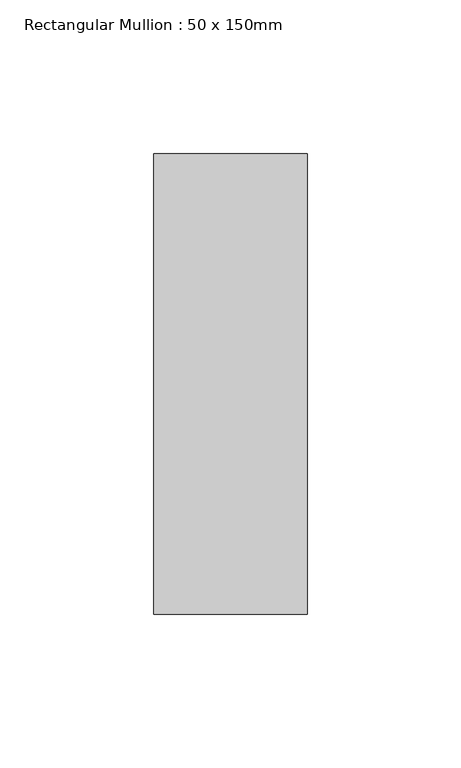
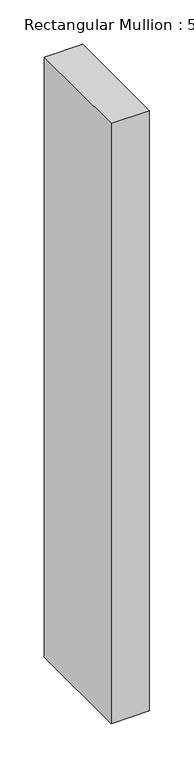
"""IFC4 building model written with IfcOpenShell, lengths in millimetres: member geometry, Rectangular Mullion : 50 x 150mm."""

import ifcopenshell
import ifcopenshell.guid

model = None  # the IFC model being written
_history = None  # IfcOwnerHistory: only IFC2X3 demands one
_inside = {}  # id of a spatial element -> (the spatial element, [elements in it])
_under = {}  # id of a project, library or spatial element -> (it, [spatial elements below it])
_declared = {}  # id of a project -> (the project, [libraries it declares])
_typed = {}  # id of a type object -> (the type object, [elements of that type])
_made_of = {}  # id of a material, layer set ... -> (it, [elements and type objects made of it])


def new_model(schema):
    """Start an empty IFC model of exactly this schema.

    Asked for "IFC4X3", IfcOpenShell would pick the latest addendum, in which some entities
    have other attributes; the version numbers below select the first issue.
    IFC2X3 requires an IfcOwnerHistory on every rooted entity: one is made here for all.
    """
    global model, _history
    if schema == "IFC4X3":
        model = ifcopenshell.file(schema_version=(4, 3, 0, 0))
    else:
        model = ifcopenshell.file(schema=schema)
    _inside.clear()
    _under.clear()
    _declared.clear()
    _typed.clear()
    _made_of.clear()
    _history = None
    if model.schema == "IFC2X3":
        org = make("IfcOrganization", Name="unknown")
        user = make(
            "IfcPersonAndOrganization",
            ThePerson=make("IfcPerson", FamilyName="unknown"),
            TheOrganization=org,
        )
        app = make(
            "IfcApplication",
            ApplicationDeveloper=org,
            Version="unknown",
            ApplicationFullName="unknown",
            ApplicationIdentifier="unknown",
        )
        _history = make(
            "IfcOwnerHistory",
            OwningUser=user,
            OwningApplication=app,
            ChangeAction="ADDED",
            CreationDate=0,
        )
    return model


def make(cls, **values):
    """One entity of the class cls with the attributes given. An attribute that is None is left unset."""
    return model.create_entity(
        cls, **{name: value for name, value in values.items() if value is not None}
    )


def rooted(cls, **values):
    """An entity with a GlobalId (a new one), such as an element, a storey or a relation."""
    return make(cls, GlobalId=ifcopenshell.guid.new(), OwnerHistory=_history, **values)


def si_unit(unit_type, name, prefix=None):
    """IfcSIUnit, for example si_unit("LENGTHUNIT", "METRE", prefix="MILLI")."""
    return make("IfcSIUnit", UnitType=unit_type, Prefix=prefix, Name=name)


def assignment(units):
    """IfcUnitAssignment: the units of a project."""
    return None if units is None else make("IfcUnitAssignment", Units=units)


def point(xyz):
    """IfcCartesianPoint."""
    return None if xyz is None else make("IfcCartesianPoint", Coordinates=xyz)


def direction(xyz):
    """IfcDirection."""
    return None if xyz is None else make("IfcDirection", DirectionRatios=xyz)


def frame(location, z_axis=None, x_axis=None):
    """IfcAxis2Placement3D, a coordinate frame: its origin and axes. An axis left out is left unset."""
    return make(
        "IfcAxis2Placement3D",
        Location=point(location),
        Axis=direction(z_axis),
        RefDirection=direction(x_axis),
    )


def origin():
    """The frame at (0, 0, 0) with its axes left unset."""
    return frame((0.0, 0.0, 0.0))


def place(relative_to, where):
    """IfcLocalPlacement: puts the frame where relative to a parent placement (None: the world)."""
    return make(
        "IfcLocalPlacement", PlacementRelTo=relative_to, RelativePlacement=where
    )


def context(
    kind, dimensions, precision=None, world=None, true_north=None, identifier=None
):
    """IfcGeometricRepresentationContext, for example the 3D "Model" context."""
    return make(
        "IfcGeometricRepresentationContext",
        ContextIdentifier=identifier,
        ContextType=kind,
        CoordinateSpaceDimension=dimensions,
        Precision=precision,
        WorldCoordinateSystem=world,
        TrueNorth=true_north,
    )


def project(units=None, contexts=None):
    """IfcProject with its units and contexts."""
    return rooted(
        "IfcProject",
        Name="project",
        RepresentationContexts=contexts,
        UnitsInContext=assignment(units),
    )


def spatial(cls, under=None, at=None, **own):
    """A site, building, storey or space (cls), placed at a placement, below another one or the project."""
    s = rooted(cls, ObjectPlacement=at, **own)
    if under is not None:
        _under.setdefault(under.id(), (under, []))[1].append(s)
    return s


def polyline(points):
    """IfcPolyline through the points."""
    return make("IfcPolyline", Points=[point(p) for p in points])


def outline(outer, holes=None, kind="AREA"):
    """IfcArbitraryClosedProfileDef: a profile drawn as a closed curve; with holes, ...WithVoids."""
    if holes is None:
        return make("IfcArbitraryClosedProfileDef", ProfileType=kind, OuterCurve=outer)
    return make(
        "IfcArbitraryProfileDefWithVoids",
        ProfileType=kind,
        OuterCurve=outer,
        InnerCurves=holes,
    )


def extrude(swept, where, along, depth):
    """IfcExtrudedAreaSolid: the profile swept, set in the frame where, extruded along a direction by depth."""
    return make(
        "IfcExtrudedAreaSolid",
        SweptArea=swept,
        Position=where,
        ExtrudedDirection=direction(along),
        Depth=depth,
    )


def shape(context_of_items, identifier, shape_type, items):
    """IfcShapeRepresentation: the items that make up one representation, for example the "Body"."""
    return make(
        "IfcShapeRepresentation",
        ContextOfItems=context_of_items,
        RepresentationIdentifier=identifier,
        RepresentationType=shape_type,
        Items=items,
    )


def source(mapping_origin, context_of_items, identifier, shape_type, items):
    """IfcRepresentationMap: a shape defined once, which mapped items show again and again."""
    return make(
        "IfcRepresentationMap",
        MappingOrigin=mapping_origin,
        MappedRepresentation=shape(context_of_items, identifier, shape_type, items),
    )


def transform(
    local_origin,
    x_axis=None,
    y_axis=None,
    z_axis=None,
    scale=None,
    scale2=None,
    scale3=None,
    uniform=True,
):
    """IfcCartesianTransformationOperator3D, or its non-uniform kind. x_axis, y_axis, z_axis: its Axis1, 2, 3."""
    if uniform:
        return make(
            "IfcCartesianTransformationOperator3D",
            Axis1=direction(x_axis),
            Axis2=direction(y_axis),
            LocalOrigin=point(local_origin),
            Scale=scale,
            Axis3=direction(z_axis),
        )
    return make(
        "IfcCartesianTransformationOperator3DnonUniform",
        Axis1=direction(x_axis),
        Axis2=direction(y_axis),
        LocalOrigin=point(local_origin),
        Scale=scale,
        Axis3=direction(z_axis),
        Scale2=scale2,
        Scale3=scale3,
    )


def mapped(mapping_source, mapping_target):
    """IfcMappedItem: shows the shape of a source again, moved by a transform."""
    return make(
        "IfcMappedItem", MappingSource=mapping_source, MappingTarget=mapping_target
    )


def made_of(thing, what):
    """Note that an element or type object is made of a material, layer set ...; save() writes the relation."""
    if what is not None:
        _made_of.setdefault(what.id(), (what, []))[1].append(thing)
    return thing


def element(
    cls,
    number,
    at=None,
    inside=None,
    cuts=None,
    type_object=None,
    material=None,
    context=None,
    identifier="Body",
    shape_type=None,
    held_by="IfcProductDefinitionShape",
    body=None,
    shapes=None,
    **own,
):
    """One element of the class cls, such as IfcWall. Its Tag is "e" and its number.

    at: its placement. inside: the storey or other place that contains it. cuts: it is an
    opening in that element (IfcRelVoidsElement). A single representation is given by context,
    identifier, shape_type and body (its items); several are given by shapes. held_by: the class
    of the entity that holds the representations. save() writes the other relations.
    """
    e = rooted(cls, Tag="e%d" % number, ObjectPlacement=at, **own)
    if body is not None:
        shapes = [shape(context, identifier, shape_type, body)]
    if shapes is not None:
        e.Representation = make(held_by, Representations=shapes)
    if inside is not None:
        _inside.setdefault(inside.id(), (inside, []))[1].append(e)
    if cuts is not None:
        rooted(
            "IfcRelVoidsElement", RelatingBuildingElement=cuts, RelatedOpeningElement=e
        )
    if type_object is not None:
        _typed.setdefault(type_object.id(), (type_object, []))[1].append(e)
    return made_of(e, material)


def aggregate(whole, parts):
    """IfcRelAggregates: a whole, such as a stair, and the parts it consists of."""
    return rooted("IfcRelAggregates", RelatingObject=whole, RelatedObjects=parts)


def save(model, path):
    """Write the relations noted so far, then the file.

    IfcRelAggregates (storeys below a building ...), IfcRelContainedInSpatialStructure (elements
    in a storey), IfcRelDefinesByType, IfcRelAssociatesMaterial and IfcRelDeclares: one each for
    every whole, place, type object, material and project.
    """
    for whole, parts in _under.values():
        aggregate(whole, parts)
    for where, things in _inside.values():
        rooted(
            "IfcRelContainedInSpatialStructure",
            RelatedElements=things,
            RelatingStructure=where,
        )
    for kind, things in _typed.values():
        rooted("IfcRelDefinesByType", RelatedObjects=things, RelatingType=kind)
    for what, things in _made_of.values():
        rooted("IfcRelAssociatesMaterial", RelatedObjects=things, RelatingMaterial=what)
    for by, libraries in _declared.values():
        rooted("IfcRelDeclares", RelatingContext=by, RelatedDefinitions=libraries)
    model.write(path)


def rectangular_mullion_50_x_150mm_4883e7f1(model_context):
    return source(origin(), model_context, "Body", "SweptSolid", [
        extrude(outline(polyline([(0.0, 75.0), (0.0, -75.0), (-50.0, -75.0), (-50.0, 75.0), (0.0, 75.0)])), frame((0.0, 0.0, -825.0), z_axis=(0.0, 0.0, 1.0), x_axis=(1.0, 0.0, 0.0)), (0.0, 0.0, 1.0), 825.0),
    ])


if __name__ == "__main__":
    model = new_model("IFC4")
    model_context = context("Model", 3, world=origin())
    ifc_project = project(units=[si_unit("LENGTHUNIT", "METRE", prefix="MILLI")], contexts=[model_context])
    site = spatial("IfcSite", under=ifc_project)
    building = spatial("IfcBuilding", under=site)
    placement = place(None, origin())
    rectangular_mullion_50_x_150mm_shape = rectangular_mullion_50_x_150mm_4883e7f1(model_context)
    element("IfcMember", 1, ObjectType="Rectangular Mullion : 50 x 150mm", at=placement, inside=building, context=model_context, shape_type="MappedRepresentation", body=[
        mapped(rectangular_mullion_50_x_150mm_shape, transform((0.0, 0.0, 0.0), x_axis=(1.0, 0.0, 0.0), y_axis=(0.0, 1.0, 0.0), z_axis=(0.0, 0.0, 1.0))),
    ])
    save(model, "model.ifc")

# Revit data of these elements
# Type "Rectangular Mullion : 50 x 150mm"
#   built-in parameter 1007304 = 0.492126 (stored number, unit not read)
#   built-in parameter 1007301 = 0.082021 (stored number, unit not read)
#   built-in parameter 1007300 = 0.082021 (stored number, unit not read)
# Element 1 (IfcMember, "Rectangular Mullion : 50 x 150mm")
#   Materials on its faces: "Metal - Aluminium"
# Materials
#   "Metal - Aluminium": class "Metal", colour RGB 247 247 247, transparency 0
